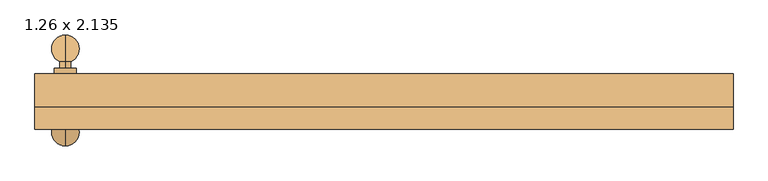
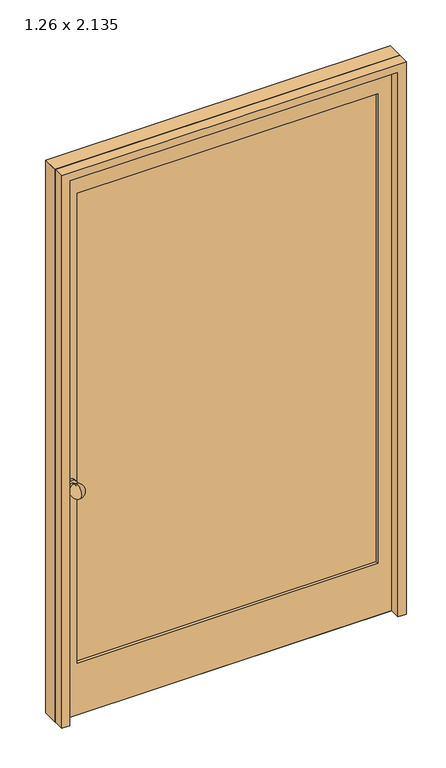
"""IFC4 building model written with IfcOpenShell, lengths in millimetres: door geometry, Eingangstür 1-flg : 1.26 x 2.135."""

from ifc_helpers import new_model, si_unit, point, frame, frame_2d, origin, place, context, project, spatial, polyline, circle_curve, ellipse_curve, trimmed, segment, composite_curve, outline, extrude, source, transform, mapped, element, save
from ifc_brep_helpers import plane_surface, cylinder_surface, revolved_surface, advanced_brep


def door_1_26_x_2_135_f7f6a525(model_context):
    return source(origin(), model_context, "Body", "SolidModel", [
        advanced_brep(
        [(-575.0, -177.6525075, 890.0), (-575.0, -225.5653859, 900.0), (-575.0, -177.6525075, 910.0), (-575.0, -165.5653859, 890.0), (-575.0, -165.5653859, 910.0), (-575.0, -165.5653859, 900.0)],
        [
            (0, 1, circle_curve(frame((-575.0, -200.5653859, 900.0), z_axis=(-1.0, 0.0, 0.0), x_axis=(0.0, -1.0, 0.0)), 25.0)),
            (1, 2, circle_curve(frame((-575.0, -200.5653859, 900.0), z_axis=(-1.0, 0.0, 0.0), x_axis=(0.0, -1.0, 0.0)), 25.0)),
            (2, 0, circle_curve(frame((-575.0, -177.6525075, 900.0), z_axis=(0.0, -1.0, 0.0), x_axis=(0.0, 0.0, 1.0)), 10.0)),
            (0, 2, circle_curve(frame((-575.0, -177.6525075, 900.0), z_axis=(0.0, -1.0, 0.0), x_axis=(0.0, 0.0, 1.0)), 10.0)),
            (3, 0),
            (2, 4),
            (4, 3, circle_curve(frame((-575.0, -165.5653859, 900.0), z_axis=(0.0, -1.0, 0.0), x_axis=(0.0, 0.0, 1.0)), 10.0)),
            (3, 4, circle_curve(frame((-575.0, -165.5653859, 900.0), z_axis=(0.0, -1.0, 0.0), x_axis=(0.0, 0.0, 1.0)), 10.0)),
            (5, 3),
            (4, 5),
        ],
        [
            revolved_surface(trimmed(ellipse_curve(frame((-575.0, -200.5653859, 900.0), z_axis=(-1.0, 0.0, 0.0), x_axis=(0.0, -1.0, 0.0)), 25.0, 25.0), [point((-575.0, -225.5653859, 900.0))], [point((-575.0, -177.6525075, 910.0))], True, "CARTESIAN"), (-575.0, 2685.9507844, 900.0), (0.0, 1.0, 0.0)),
            cylinder_surface(frame((-575.0, 2685.9507844, 900.0), z_axis=(0.0, 1.0, 0.0), x_axis=(0.0, 0.0, 1.0)), 10.0),
            plane_surface(frame((-575.0, -165.5653859, 900.0), z_axis=(0.0, 1.0, 0.0), x_axis=(0.0, 0.0, 1.0))),
        ],
        [
            (0, [[1, 2, 3]]),
            (0, [[-2, -1, 4]]),
            (1, [[5, -3, 6, 7]]),
            (1, [[-6, -4, -5, 8]]),
            (2, [[9, -7, 10]]),
            (2, [[-10, -8, -9]]),
        ],
    ),
        extrude(outline(composite_curve([segment(trimmed(circle_curve(frame_2d((900.0, -575.0)), 20.0), [point((900.0, -555.0))], [point((900.0, -595.0))], False, "CARTESIAN"), True, "CONTINUOUS"), segment(trimmed(circle_curve(frame_2d((900.0, -575.0)), 20.0), [point((900.0, -595.0))], [point((900.0, -555.0))], False, "CARTESIAN"), True, "CONTINUOUS")], self_intersect=False)), frame((0.0, -165.5653859, 0.0), z_axis=(0.0, 1.0, 0.0), x_axis=(0.0, 0.0, 1.0)), (0.0, 0.0, 1.0), 10.0),
        advanced_brep(
        [(-575.0, -73.4782644, 890.0), (-575.0, -73.4782644, 910.0), (-575.0, -25.5653859, 900.0), (-575.0, -85.5653859, 890.0), (-575.0, -85.5653859, 910.0), (-575.0, -85.5653859, 900.0)],
        [
            (0, 1, circle_curve(frame((-575.0, -73.4782644, 900.0), z_axis=(0.0, 1.0, 0.0), x_axis=(0.0, 0.0, 1.0)), 10.0)),
            (1, 2, circle_curve(frame((-575.0, -50.5653859, 900.0), z_axis=(-1.0, 0.0, 0.0), x_axis=(0.0, 1.0, 0.0)), 25.0)),
            (2, 0, circle_curve(frame((-575.0, -50.5653859, 900.0), z_axis=(-1.0, 0.0, 0.0), x_axis=(0.0, 1.0, 0.0)), 25.0)),
            (1, 0, circle_curve(frame((-575.0, -73.4782644, 900.0), z_axis=(0.0, 1.0, 0.0), x_axis=(0.0, 0.0, 1.0)), 10.0)),
            (3, 4, circle_curve(frame((-575.0, -85.5653859, 900.0), z_axis=(0.0, 1.0, 0.0), x_axis=(0.0, 0.0, 1.0)), 10.0)),
            (4, 1),
            (0, 3),
            (4, 3, circle_curve(frame((-575.0, -85.5653859, 900.0), z_axis=(0.0, 1.0, 0.0), x_axis=(0.0, 0.0, 1.0)), 10.0)),
            (5, 4),
            (3, 5),
        ],
        [
            revolved_surface(trimmed(ellipse_curve(frame((-575.0, -50.5653859, 900.0), z_axis=(1.0, 0.0, 0.0), x_axis=(0.0, 1.0, 0.0)), 25.0, 25.0), [point((-575.0, -25.5653859, 900.0))], [point((-575.0, -73.4782644, 910.0))], True, "CARTESIAN"), (-575.0, -2937.0815562, 900.0), (0.0, -1.0, 0.0)),
            cylinder_surface(frame((-575.0, -2937.0815562, 900.0), z_axis=(0.0, -1.0, 0.0), x_axis=(0.0, 0.0, 1.0)), 10.0),
            plane_surface(frame((-575.0, -85.5653859, 900.0), z_axis=(0.0, -1.0, 0.0), x_axis=(0.0, 0.0, 1.0))),
        ],
        [
            (0, [[1, 2, 3]]),
            (0, [[4, -3, -2]]),
            (1, [[5, 6, -1, 7]]),
            (1, [[8, -7, -4, -6]]),
            (2, [[9, -5, 10]]),
            (2, [[-10, -8, -9]]),
        ],
    ),
        extrude(outline(composite_curve([segment(trimmed(circle_curve(frame_2d((900.0, -575.0)), 20.0), [point((900.0, -555.0))], [point((900.0, -595.0))], False, "CARTESIAN"), True, "CONTINUOUS"), segment(trimmed(circle_curve(frame_2d((900.0, -575.0)), 20.0), [point((900.0, -595.0))], [point((900.0, -555.0))], False, "CARTESIAN"), True, "CONTINUOUS")], self_intersect=False)), frame((0.0, -95.5653859, 0.0), z_axis=(0.0, 1.0, 0.0), x_axis=(0.0, 0.0, 1.0)), (0.0, 0.0, 1.0), 10.0),
        extrude(outline(polyline([(550.0, -143.9440021), (-550.0, -143.9440021), (-550.0, -118.9440021), (550.0, -118.9440021), (550.0, -143.9440021)])), frame((0.0, 0.0, 200.0), z_axis=(0.0, 0.0, 1.0), x_axis=(1.0, 0.0, 0.0)), (0.0, 0.0, 1.0), 1815.0),
        extrude(outline(polyline([(2135.0, 630.0), (2135.0, -630.0), (0.0, -630.0), (0.0, 630.0), (2135.0, 630.0)]), holes=[polyline([(2015.0, -550.0), (2015.0, 550.0), (200.0, 550.0), (200.0, -550.0), (2015.0, -550.0)])]), frame((0.0, -155.5653859, 0.0), z_axis=(0.0, 1.0, 0.0), x_axis=(0.0, 0.0, 1.0)), (0.0, 0.0, 1.0), 60.0),
        extrude(outline(polyline([(0.0, 600.0), (0.0, 630.0), (2135.0, 630.0), (2135.0, -630.0), (0.0, -630.0), (0.0, -600.0), (2105.0, -600.0), (2105.0, 600.0), (0.0, 600.0)])), frame((0.0, -195.5653859, 0.0), z_axis=(0.0, 1.0, 0.0), x_axis=(0.0, 0.0, 1.0)), (0.0, 0.0, 1.0), 100.0),
        extrude(outline(polyline([(2105.0, -600.0), (0.0, -600.0), (0.0, 600.0), (2105.0, 600.0), (2105.0, -600.0)]), holes=[polyline([(2015.0, -550.0), (2015.0, 550.0), (200.0, 550.0), (200.0, -550.0), (2015.0, -550.0)])]), frame((0.0, -155.5653859, 0.0), z_axis=(0.0, 1.0, 0.0), x_axis=(0.0, 0.0, 1.0)), (0.0, 0.0, 1.0), 60.0),
    ])


if __name__ == "__main__":
    model = new_model("IFC4")
    model_context = context("Model", 3, world=origin())
    ifc_project = project(units=[si_unit("LENGTHUNIT", "METRE", prefix="MILLI")], contexts=[model_context])
    site = spatial("IfcSite", under=ifc_project)
    building = spatial("IfcBuilding", under=site)
    placement = place(None, origin())
    door_1_26_x_2_135_shape = door_1_26_x_2_135_f7f6a525(model_context)
    element("IfcDoor", 1, ObjectType="Eingangstür 1-flg : 1.26 x 2.135", at=placement, inside=building, context=model_context, shape_type="MappedRepresentation", body=[
        mapped(door_1_26_x_2_135_shape, transform((0.0, 0.0, 0.0), x_axis=(1.0, 0.0, 0.0), y_axis=(0.0, 1.0, 0.0), z_axis=(0.0, 0.0, 1.0))),
    ])
    save(model, "model.ifc")

# Revit data of these elements
# Type "Eingangstür 1-flg : 1.26 x 2.135"
#   Type Mark = "22"
#   Operation = "SingleSwingLeft"
#   Construction Type Id = "opn-d40"
#   Keynote = "16.03"
#   Analytic Construction = "Metall, Glasfaserkern, Sturmtür"
#   Stärke Futter = 0.030 m
#   Heat Transfer Coefficient (U) = 2.0838 W/(m²·K)
#   Rough Width = 1.260 m
#   Rahmentiefe = 0.060 m
#   Rahmenhöhe - oben = 0.120 m
#   Rahmenbreite unten = 0.200 m
#   Rahmenbreite = 0.080 m
#   Rough Height [instance default] = 2.235 m
#   LichteBreite = 1.100 m
#   Höhe Türgriff = 0.900 m
#   Height = 2.135 m
#   Fußbodenaufbau [instance default] = 0.100 m
#   Einbautiefe (von außen) [instance default] = 0.080 m
#   Width = 1.260 m
#   Sichtbarkeit Sturzlinien [instance default] = yes
#   Function = 1
#   Türgriff auswählen [instance default] = element 474727
#   Türgriff [instance default] = none
#   Türblatt Füllelement [instance default] = Holz - Birke
#   Türflügel [instance default] = none
#   Rahmen/Pfosten [instance default] = none
#   Visual Light Transmittance = 0
#   Solar Heat Gain Coefficient = 0
#   Wall Closure = (empty or 0)
# Element 1 (IfcDoor, "Eingangstür 1-flg : 1.26 x 2.135")
#   Rough Height = 2.135 m
#   Fußbodenaufbau = 0.000 m
#   Einbautiefe (von außen) = 0.000 m
#   Türblatt Füllelement = Metall - Edelstahl, poliert
#   Materials on its faces: "Holz - Birke", "Metall - Chrom", "Metall - Edelstahl, poliert"
# Materials
#   "Holz - Birke": class "Holz", colour RGB 213 164 103, transparency 0, Cost = 0
#   "Metall - Chrom": class "Metall", colour RGB 247 247 247, transparency 0, Cost = 0
#   "Metall - Edelstahl, poliert": class "Metall", colour RGB 192 192 192, transparency 0, Cost = 0
